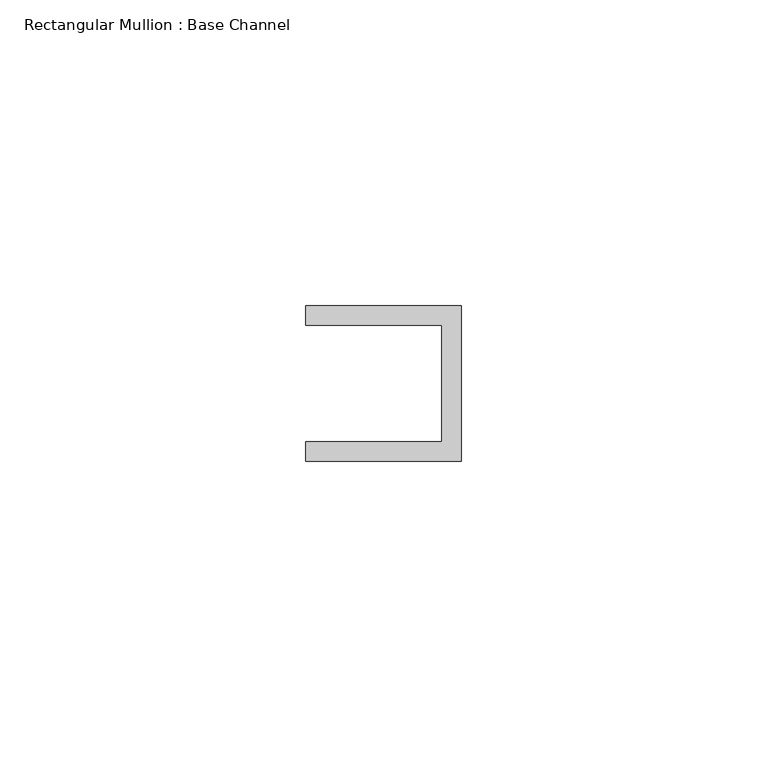
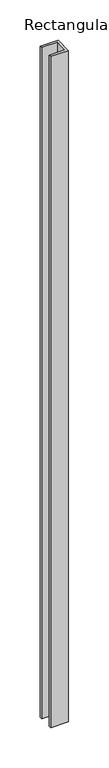
"""IFC4 building model written with IfcOpenShell, lengths in millimetres: member geometry, Rectangular Mullion : Base Channel."""

import ifcopenshell
import ifcopenshell.guid

model = None  # the IFC model being written
_history = None  # IfcOwnerHistory: only IFC2X3 demands one
_inside = {}  # id of a spatial element -> (the spatial element, [elements in it])
_under = {}  # id of a project, library or spatial element -> (it, [spatial elements below it])
_declared = {}  # id of a project -> (the project, [libraries it declares])
_typed = {}  # id of a type object -> (the type object, [elements of that type])
_made_of = {}  # id of a material, layer set ... -> (it, [elements and type objects made of it])


def new_model(schema):
    """Start an empty IFC model of exactly this schema.

    Asked for "IFC4X3", IfcOpenShell would pick the latest addendum, in which some entities
    have other attributes; the version numbers below select the first issue.
    IFC2X3 requires an IfcOwnerHistory on every rooted entity: one is made here for all.
    """
    global model, _history
    if schema == "IFC4X3":
        model = ifcopenshell.file(schema_version=(4, 3, 0, 0))
    else:
        model = ifcopenshell.file(schema=schema)
    _inside.clear()
    _under.clear()
    _declared.clear()
    _typed.clear()
    _made_of.clear()
    _history = None
    if model.schema == "IFC2X3":
        org = make("IfcOrganization", Name="unknown")
        user = make(
            "IfcPersonAndOrganization",
            ThePerson=make("IfcPerson", FamilyName="unknown"),
            TheOrganization=org,
        )
        app = make(
            "IfcApplication",
            ApplicationDeveloper=org,
            Version="unknown",
            ApplicationFullName="unknown",
            ApplicationIdentifier="unknown",
        )
        _history = make(
            "IfcOwnerHistory",
            OwningUser=user,
            OwningApplication=app,
            ChangeAction="ADDED",
            CreationDate=0,
        )
    return model


def make(cls, **values):
    """One entity of the class cls with the attributes given. An attribute that is None is left unset."""
    return model.create_entity(
        cls, **{name: value for name, value in values.items() if value is not None}
    )


def rooted(cls, **values):
    """An entity with a GlobalId (a new one), such as an element, a storey or a relation."""
    return make(cls, GlobalId=ifcopenshell.guid.new(), OwnerHistory=_history, **values)


def si_unit(unit_type, name, prefix=None):
    """IfcSIUnit, for example si_unit("LENGTHUNIT", "METRE", prefix="MILLI")."""
    return make("IfcSIUnit", UnitType=unit_type, Prefix=prefix, Name=name)


def assignment(units):
    """IfcUnitAssignment: the units of a project."""
    return None if units is None else make("IfcUnitAssignment", Units=units)


def point(xyz):
    """IfcCartesianPoint."""
    return None if xyz is None else make("IfcCartesianPoint", Coordinates=xyz)


def direction(xyz):
    """IfcDirection."""
    return None if xyz is None else make("IfcDirection", DirectionRatios=xyz)


def frame(location, z_axis=None, x_axis=None):
    """IfcAxis2Placement3D, a coordinate frame: its origin and axes. An axis left out is left unset."""
    return make(
        "IfcAxis2Placement3D",
        Location=point(location),
        Axis=direction(z_axis),
        RefDirection=direction(x_axis),
    )


def origin():
    """The frame at (0, 0, 0) with its axes left unset."""
    return frame((0.0, 0.0, 0.0))


def place(relative_to, where):
    """IfcLocalPlacement: puts the frame where relative to a parent placement (None: the world)."""
    return make(
        "IfcLocalPlacement", PlacementRelTo=relative_to, RelativePlacement=where
    )


def context(
    kind, dimensions, precision=None, world=None, true_north=None, identifier=None
):
    """IfcGeometricRepresentationContext, for example the 3D "Model" context."""
    return make(
        "IfcGeometricRepresentationContext",
        ContextIdentifier=identifier,
        ContextType=kind,
        CoordinateSpaceDimension=dimensions,
        Precision=precision,
        WorldCoordinateSystem=world,
        TrueNorth=true_north,
    )


def project(units=None, contexts=None):
    """IfcProject with its units and contexts."""
    return rooted(
        "IfcProject",
        Name="project",
        RepresentationContexts=contexts,
        UnitsInContext=assignment(units),
    )


def spatial(cls, under=None, at=None, **own):
    """A site, building, storey or space (cls), placed at a placement, below another one or the project."""
    s = rooted(cls, ObjectPlacement=at, **own)
    if under is not None:
        _under.setdefault(under.id(), (under, []))[1].append(s)
    return s


def polyline(points):
    """IfcPolyline through the points."""
    return make("IfcPolyline", Points=[point(p) for p in points])


def outline(outer, holes=None, kind="AREA"):
    """IfcArbitraryClosedProfileDef: a profile drawn as a closed curve; with holes, ...WithVoids."""
    if holes is None:
        return make("IfcArbitraryClosedProfileDef", ProfileType=kind, OuterCurve=outer)
    return make(
        "IfcArbitraryProfileDefWithVoids",
        ProfileType=kind,
        OuterCurve=outer,
        InnerCurves=holes,
    )


def extrude(swept, where, along, depth):
    """IfcExtrudedAreaSolid: the profile swept, set in the frame where, extruded along a direction by depth."""
    return make(
        "IfcExtrudedAreaSolid",
        SweptArea=swept,
        Position=where,
        ExtrudedDirection=direction(along),
        Depth=depth,
    )


def shape(context_of_items, identifier, shape_type, items):
    """IfcShapeRepresentation: the items that make up one representation, for example the "Body"."""
    return make(
        "IfcShapeRepresentation",
        ContextOfItems=context_of_items,
        RepresentationIdentifier=identifier,
        RepresentationType=shape_type,
        Items=items,
    )


def source(mapping_origin, context_of_items, identifier, shape_type, items):
    """IfcRepresentationMap: a shape defined once, which mapped items show again and again."""
    return make(
        "IfcRepresentationMap",
        MappingOrigin=mapping_origin,
        MappedRepresentation=shape(context_of_items, identifier, shape_type, items),
    )


def transform(
    local_origin,
    x_axis=None,
    y_axis=None,
    z_axis=None,
    scale=None,
    scale2=None,
    scale3=None,
    uniform=True,
):
    """IfcCartesianTransformationOperator3D, or its non-uniform kind. x_axis, y_axis, z_axis: its Axis1, 2, 3."""
    if uniform:
        return make(
            "IfcCartesianTransformationOperator3D",
            Axis1=direction(x_axis),
            Axis2=direction(y_axis),
            LocalOrigin=point(local_origin),
            Scale=scale,
            Axis3=direction(z_axis),
        )
    return make(
        "IfcCartesianTransformationOperator3DnonUniform",
        Axis1=direction(x_axis),
        Axis2=direction(y_axis),
        LocalOrigin=point(local_origin),
        Scale=scale,
        Axis3=direction(z_axis),
        Scale2=scale2,
        Scale3=scale3,
    )


def mapped(mapping_source, mapping_target):
    """IfcMappedItem: shows the shape of a source again, moved by a transform."""
    return make(
        "IfcMappedItem", MappingSource=mapping_source, MappingTarget=mapping_target
    )


def made_of(thing, what):
    """Note that an element or type object is made of a material, layer set ...; save() writes the relation."""
    if what is not None:
        _made_of.setdefault(what.id(), (what, []))[1].append(thing)
    return thing


def element(
    cls,
    number,
    at=None,
    inside=None,
    cuts=None,
    type_object=None,
    material=None,
    context=None,
    identifier="Body",
    shape_type=None,
    held_by="IfcProductDefinitionShape",
    body=None,
    shapes=None,
    **own,
):
    """One element of the class cls, such as IfcWall. Its Tag is "e" and its number.

    at: its placement. inside: the storey or other place that contains it. cuts: it is an
    opening in that element (IfcRelVoidsElement). A single representation is given by context,
    identifier, shape_type and body (its items); several are given by shapes. held_by: the class
    of the entity that holds the representations. save() writes the other relations.
    """
    e = rooted(cls, Tag="e%d" % number, ObjectPlacement=at, **own)
    if body is not None:
        shapes = [shape(context, identifier, shape_type, body)]
    if shapes is not None:
        e.Representation = make(held_by, Representations=shapes)
    if inside is not None:
        _inside.setdefault(inside.id(), (inside, []))[1].append(e)
    if cuts is not None:
        rooted(
            "IfcRelVoidsElement", RelatingBuildingElement=cuts, RelatedOpeningElement=e
        )
    if type_object is not None:
        _typed.setdefault(type_object.id(), (type_object, []))[1].append(e)
    return made_of(e, material)


def aggregate(whole, parts):
    """IfcRelAggregates: a whole, such as a stair, and the parts it consists of."""
    return rooted("IfcRelAggregates", RelatingObject=whole, RelatedObjects=parts)


def save(model, path):
    """Write the relations noted so far, then the file.

    IfcRelAggregates (storeys below a building ...), IfcRelContainedInSpatialStructure (elements
    in a storey), IfcRelDefinesByType, IfcRelAssociatesMaterial and IfcRelDeclares: one each for
    every whole, place, type object, material and project.
    """
    for whole, parts in _under.values():
        aggregate(whole, parts)
    for where, things in _inside.values():
        rooted(
            "IfcRelContainedInSpatialStructure",
            RelatedElements=things,
            RelatingStructure=where,
        )
    for kind, things in _typed.values():
        rooted("IfcRelDefinesByType", RelatedObjects=things, RelatingType=kind)
    for what, things in _made_of.values():
        rooted("IfcRelAssociatesMaterial", RelatedObjects=things, RelatingMaterial=what)
    for by, libraries in _declared.values():
        rooted("IfcRelDeclares", RelatingContext=by, RelatedDefinitions=libraries)
    model.write(path)


def rectangular_mullion_base_channel_d92864c2(model_context):
    return source(origin(), model_context, "Body", "SweptSolid", [
        extrude(outline(polyline([(0.0, -12.7), (-25.4, -12.7), (-25.4, -9.525), (-3.175, -9.525), (-3.175, 9.525), (-25.4, 9.525), (-25.4, 12.7), (0.0, 12.7), (0.0, -12.7)])), frame((0.0, 0.0, -1016.0), z_axis=(0.0, 0.0, 1.0), x_axis=(1.0, 0.0, 0.0)), (0.0, 0.0, 1.0), 1016.0),
    ])


if __name__ == "__main__":
    model = new_model("IFC4")
    model_context = context("Model", 3, world=origin())
    ifc_project = project(units=[si_unit("LENGTHUNIT", "METRE", prefix="MILLI")], contexts=[model_context])
    site = spatial("IfcSite", under=ifc_project)
    building = spatial("IfcBuilding", under=site)
    placement = place(None, origin())
    rectangular_mullion_base_channel_shape = rectangular_mullion_base_channel_d92864c2(model_context)
    element("IfcMember", 1, ObjectType="Rectangular Mullion : Base Channel", at=placement, inside=building, context=model_context, shape_type="MappedRepresentation", body=[
        mapped(rectangular_mullion_base_channel_shape, transform((0.0, 0.0, 0.0), x_axis=(1.0, 0.0, 0.0), y_axis=(0.0, 1.0, 0.0), z_axis=(0.0, 0.0, 1.0))),
    ])
    save(model, "model.ifc")

# Revit data of these elements
# Type "Rectangular Mullion : Base Channel"
#   built-in parameter 1007322 = 0.0833333 (stored number, unit not read)
#   built-in parameter 1007321 = 0.0416667 (stored number, unit not read)
#   built-in parameter 1007320 = -0.03125 (stored number, unit not read)
# Element 1 (IfcMember, "Rectangular Mullion : Base Channel")
#   Materials on its faces: "ALUM"
# Materials
#   "ALUM": class "Generic", colour RGB 157 157 157, transparency 0, Cost = 0
